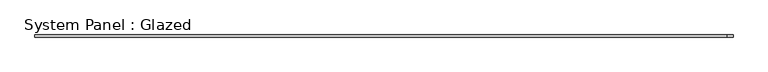
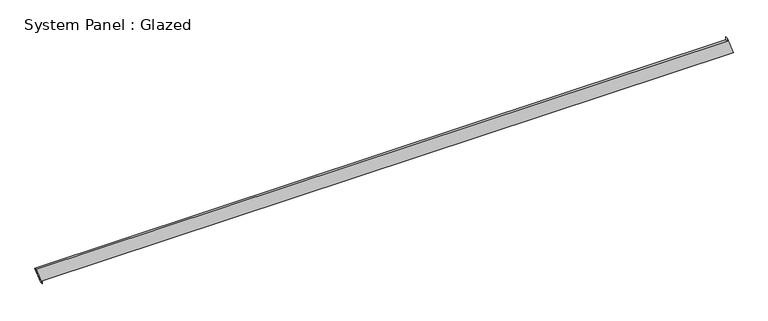
"""IFC4 building model written with IfcOpenShell, lengths in millimetres: plate geometry, System Panel : Glazed."""

from ifc_helpers import new_model, si_unit, frame, origin, place, context, project, spatial, polyline, outline, extrude, source, transform, mapped, element, save


def system_panel_glazed_c8b449c2(model_context):
    return source(origin(), model_context, "Body", "SweptSolid", [
        extrude(outline(polyline([(0.0, -3958.4846082), (35.3553391, -3958.4846082), (35.3553391, 4028.1165848), (235.3243648, 3958.401505), (199.9690258, 3958.4013511), (200.0037824, -4028.1165848), (0.0, -3958.4846082)])), frame((0.0, -49.5, 0.0), z_axis=(0.0, 1.0, 0.0), x_axis=(0.0, 0.0, 1.0)), (0.0, 0.0, 1.0), 25.0),
    ])


if __name__ == "__main__":
    model = new_model("IFC4")
    model_context = context("Model", 3, world=origin())
    ifc_project = project(units=[si_unit("LENGTHUNIT", "METRE", prefix="MILLI")], contexts=[model_context])
    site = spatial("IfcSite", under=ifc_project)
    building = spatial("IfcBuilding", under=site)
    placement = place(None, origin())
    system_panel_glazed_shape = system_panel_glazed_c8b449c2(model_context)
    element("IfcPlate", 1, ObjectType="System Panel : Glazed", at=placement, inside=building, context=model_context, shape_type="MappedRepresentation", body=[
        mapped(system_panel_glazed_shape, transform((0.0, 0.0, 0.0), x_axis=(1.0, 0.0, 0.0), y_axis=(0.0, 1.0, 0.0), z_axis=(0.0, 0.0, 1.0))),
    ])
    save(model, "model.ifc")

# Revit data of these elements
# Element 1 (IfcPlate, "System Panel : Glazed")
#   Materials on its faces: "Glass"
# Materials
#   "Glass": class "Glass", colour RGB 218 227 224, transparency 0.85, Description = "Soda Lime Glass", Cost = 0
